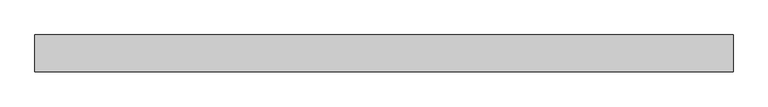
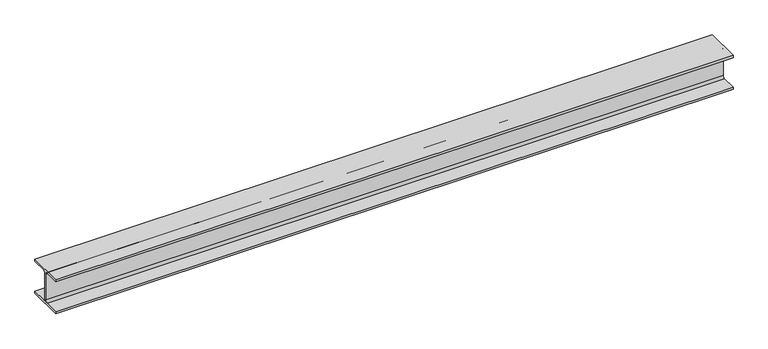
"""IFC4 building model written with IfcOpenShell, lengths in millimetres: beam geometry, 0912_Steel Framing_H-KSD3502 : H_SB_ASB_H-200x200x8x12."""

from ifc_helpers import new_model, si_unit, point, frame, frame_2d, origin, place, context, project, spatial, polyline, circle_curve, trimmed, segment, composite_curve, outline, extrude, source, transform, mapped, element, save


def beam_b60be60a(model_context):
    return source(origin(), model_context, "Body", "SweptSolid", [
        extrude(outline(composite_curve([segment(polyline([(100.0, -88.0), (100.0, -100.0), (-100.0, -100.0), (-100.0, -88.0), (-17.0, -88.0)]), True, "CONTINUOUS"), segment(trimmed(circle_curve(frame_2d((-17.0, -75.0)), 13.0), [point((-17.0, -88.0))], [point((-4.0, -75.0))], True, "CARTESIAN"), True, "CONTINUOUS"), segment(polyline([(-4.0, -75.0), (-4.0, 75.0)]), True, "CONTINUOUS"), segment(trimmed(circle_curve(frame_2d((-17.0, 75.0)), 13.0), [point((-4.0, 75.0))], [point((-17.0, 88.0))], True, "CARTESIAN"), True, "CONTINUOUS"), segment(polyline([(-17.0, 88.0), (-100.0, 88.0), (-100.0, 100.0), (100.0, 100.0), (100.0, 88.0), (17.0, 88.0)]), True, "CONTINUOUS"), segment(trimmed(circle_curve(frame_2d((17.0, 75.0)), 13.0), [point((17.0, 88.0))], [point((4.0, 75.0))], True, "CARTESIAN"), True, "CONTINUOUS"), segment(polyline([(4.0, 75.0), (4.0, -75.0)]), True, "CONTINUOUS"), segment(trimmed(circle_curve(frame_2d((17.0, -75.0)), 13.0), [point((4.0, -75.0))], [point((17.0, -88.0))], True, "CARTESIAN"), True, "CONTINUOUS"), segment(polyline([(17.0, -88.0), (100.0, -88.0)]), True, "CONTINUOUS")], self_intersect=False)), frame((-1977.1945946, 0.0, 0.0), z_axis=(1.0, 0.0, 0.0), x_axis=(0.0, 1.0, 0.0)), (0.0, 0.0, 1.0), 3777.5770244),
    ])


if __name__ == "__main__":
    model = new_model("IFC4")
    model_context = context("Model", 3, world=origin())
    ifc_project = project(units=[si_unit("LENGTHUNIT", "METRE", prefix="MILLI")], contexts=[model_context])
    site = spatial("IfcSite", under=ifc_project)
    building = spatial("IfcBuilding", under=site)
    placement = place(None, origin())
    beam_shape = beam_b60be60a(model_context)
    element("IfcBeam", 1, ObjectType="0912_Steel Framing_H-KSD3502 : H_SB_ASB_H-200x200x8x12", at=placement, inside=building, context=model_context, shape_type="MappedRepresentation", body=[
        mapped(beam_shape, transform((0.0, 0.0, 0.0), x_axis=(1.0, 0.0, 0.0), y_axis=(0.0, 1.0, 0.0), z_axis=(0.0, 0.0, 1.0))),
    ])
    save(model, "model.ifc")

# Revit data of these elements
# Type "0912_Steel Framing_H-KSD3502 : H_SB_ASB_H-200x200x8x12"
#   H_WM Code_1 = "S01AA002-00001 | Main Steel Structure Fabrication Work | Shelter/Building | Medium Steel - Standard (90KG/M>Weight≥30KG/M) | Material: (   )"
#   H_WM Code_2 = "S03AA028-00001 | Main Steel Structure Erection Work | Shelter/Building | Medium Steel (90KG/M>Weight≥30KG/M) | Material: (   )"
#   H_WM Code_3 = "S01AA010-00001 | Main Steel Structure Fabrication Work | Shelter/Building | Steel Painting/Coating | for Non-Fireproofed Steel Surface, Surface Preparation, Primer, Second & Final Coat | Material: (   )"
#   H_Q'ty Cal Type Tag = "SB-Q2"
#   Width = 20.0 cm
#   Web Thickness = 0.8 cm
#   Web Fillet = 1.3 cm
#   Warping Constant = 141000.0 cm⁶
#   W = 0
#   Torsional Moment of Inertia = 26.2485 cm⁴
#   Section Area = 63.53 cm²
#   Plastic Modulus weak axis = 244.0 cm³
#   Plastic Modulus strong axis = 525.0 cm³
#   Perimeter = 1.16 m²/m
#   Nominal Weight = 49.90 kgf/m
#   Moment of Inertia weak axis = 1600.00 cm⁴
#   Moment of Inertia strong axis = 4720.00 cm⁴
#   Height = 20.0 cm
#   Flange Thickness = 1.2 cm
#   Elastic Modulus weak axis = 160.0 cm³
#   Elastic Modulus strong axis = 472.0 cm³
#   Centroid Vertical = 10.0 cm
#   Centroid Horizontal = 10.0 cm
#   Ix = 47200000
#   Length [instance default] = 1.5240 m
#   Zx = 525000
#   b = 0.2000 m
#   h = 0.2000 m
#   r = 0.0130 m
#   s = 0.0080 m
#   t = 0.0120 m
#   A = 0.006353 m²
#   Structural Material [instance default] = Steel, 45-345
#   Assembly Code = ""
# Element 1 (IfcBeam, "0912_Steel Framing_H-KSD3502 : H_SB_ASB_H-200x200x8x12")
#   Structural Material = none
# Materials
#   "Steel, 45-345": class "Metal", colour RGB 189 187 185, transparency 0, Description = "Steel 345 MPa", Cost = 0
